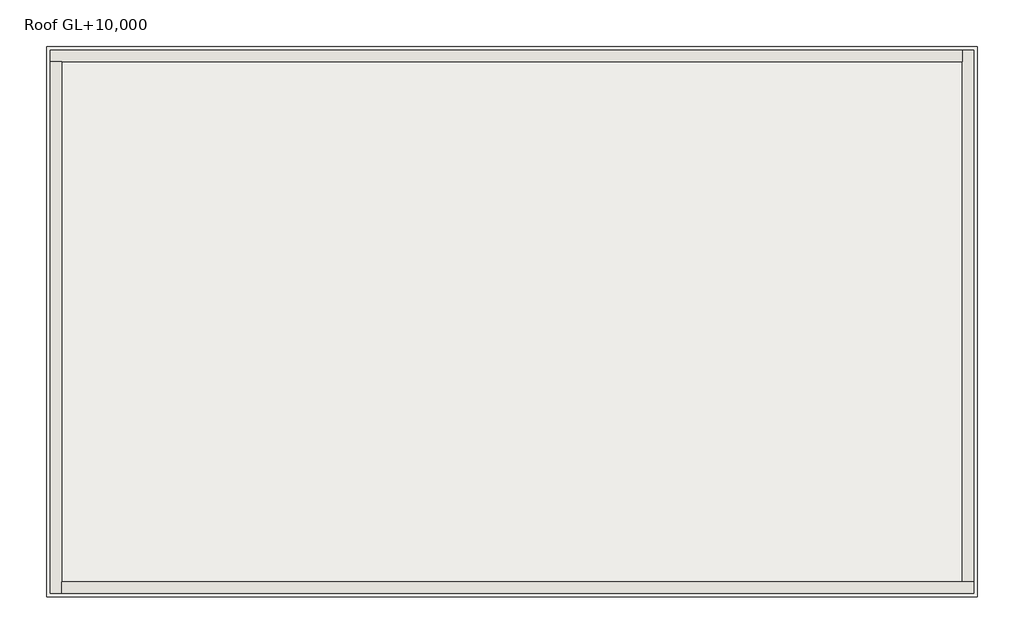
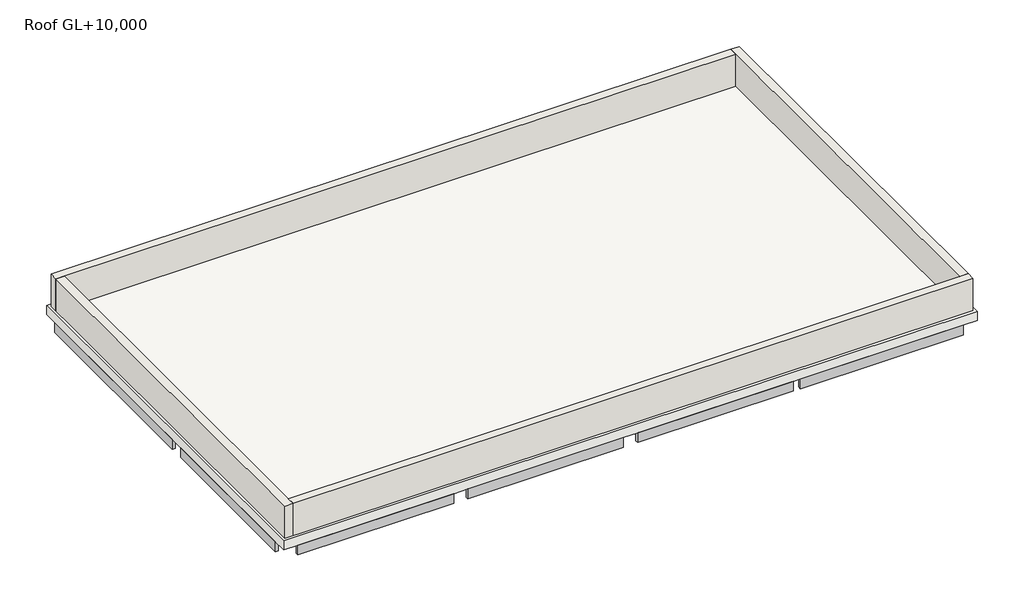
# One storey: 22 beams, 4 walls, 1 roof.
"""IFC4 building model written with IfcOpenShell, lengths in millimetres."""

import ifcopenshell
import ifcopenshell.guid

model = None  # the IFC model being written
_history = None  # IfcOwnerHistory: only IFC2X3 demands one
_inside = {}  # id of a spatial element -> (the spatial element, [elements in it])
_under = {}  # id of a project, library or spatial element -> (it, [spatial elements below it])
_declared = {}  # id of a project -> (the project, [libraries it declares])
_typed = {}  # id of a type object -> (the type object, [elements of that type])
_made_of = {}  # id of a material, layer set ... -> (it, [elements and type objects made of it])


def new_model(schema):
    """Start an empty IFC model of exactly this schema.

    Asked for "IFC4X3", IfcOpenShell would pick the latest addendum, in which some entities
    have other attributes; the version numbers below select the first issue.
    IFC2X3 requires an IfcOwnerHistory on every rooted entity: one is made here for all.
    """
    global model, _history
    if schema == "IFC4X3":
        model = ifcopenshell.file(schema_version=(4, 3, 0, 0))
    else:
        model = ifcopenshell.file(schema=schema)
    _inside.clear()
    _under.clear()
    _declared.clear()
    _typed.clear()
    _made_of.clear()
    _history = None
    if model.schema == "IFC2X3":
        org = make("IfcOrganization", Name="unknown")
        user = make(
            "IfcPersonAndOrganization",
            ThePerson=make("IfcPerson", FamilyName="unknown"),
            TheOrganization=org,
        )
        app = make(
            "IfcApplication",
            ApplicationDeveloper=org,
            Version="unknown",
            ApplicationFullName="unknown",
            ApplicationIdentifier="unknown",
        )
        _history = make(
            "IfcOwnerHistory",
            OwningUser=user,
            OwningApplication=app,
            ChangeAction="ADDED",
            CreationDate=0,
        )
    return model


def make(cls, **values):
    """One entity of the class cls with the attributes given. An attribute that is None is left unset."""
    return model.create_entity(
        cls, **{name: value for name, value in values.items() if value is not None}
    )


def rooted(cls, **values):
    """An entity with a GlobalId (a new one), such as an element, a storey or a relation."""
    return make(cls, GlobalId=ifcopenshell.guid.new(), OwnerHistory=_history, **values)


def si_unit(unit_type, name, prefix=None):
    """IfcSIUnit, for example si_unit("LENGTHUNIT", "METRE", prefix="MILLI")."""
    return make("IfcSIUnit", UnitType=unit_type, Prefix=prefix, Name=name)


def assignment(units):
    """IfcUnitAssignment: the units of a project."""
    return None if units is None else make("IfcUnitAssignment", Units=units)


def point(xyz):
    """IfcCartesianPoint."""
    return None if xyz is None else make("IfcCartesianPoint", Coordinates=xyz)


def direction(xyz):
    """IfcDirection."""
    return None if xyz is None else make("IfcDirection", DirectionRatios=xyz)


def frame(location, z_axis=None, x_axis=None):
    """IfcAxis2Placement3D, a coordinate frame: its origin and axes. An axis left out is left unset."""
    return make(
        "IfcAxis2Placement3D",
        Location=point(location),
        Axis=direction(z_axis),
        RefDirection=direction(x_axis),
    )


def origin():
    """The frame at (0, 0, 0) with its axes left unset."""
    return frame((0.0, 0.0, 0.0))


def place(relative_to, where):
    """IfcLocalPlacement: puts the frame where relative to a parent placement (None: the world)."""
    return make(
        "IfcLocalPlacement", PlacementRelTo=relative_to, RelativePlacement=where
    )


def context(
    kind, dimensions, precision=None, world=None, true_north=None, identifier=None
):
    """IfcGeometricRepresentationContext, for example the 3D "Model" context."""
    return make(
        "IfcGeometricRepresentationContext",
        ContextIdentifier=identifier,
        ContextType=kind,
        CoordinateSpaceDimension=dimensions,
        Precision=precision,
        WorldCoordinateSystem=world,
        TrueNorth=true_north,
    )


def project(units=None, contexts=None):
    """IfcProject with its units and contexts."""
    return rooted(
        "IfcProject",
        Name="project",
        RepresentationContexts=contexts,
        UnitsInContext=assignment(units),
    )


def spatial(cls, under=None, at=None, **own):
    """A site, building, storey or space (cls), placed at a placement, below another one or the project."""
    s = rooted(cls, ObjectPlacement=at, **own)
    if under is not None:
        _under.setdefault(under.id(), (under, []))[1].append(s)
    return s


def polyline(points):
    """IfcPolyline through the points."""
    return make("IfcPolyline", Points=[point(p) for p in points])


def outline(outer, holes=None, kind="AREA"):
    """IfcArbitraryClosedProfileDef: a profile drawn as a closed curve; with holes, ...WithVoids."""
    if holes is None:
        return make("IfcArbitraryClosedProfileDef", ProfileType=kind, OuterCurve=outer)
    return make(
        "IfcArbitraryProfileDefWithVoids",
        ProfileType=kind,
        OuterCurve=outer,
        InnerCurves=holes,
    )


def extrude(swept, where, along, depth):
    """IfcExtrudedAreaSolid: the profile swept, set in the frame where, extruded along a direction by depth."""
    return make(
        "IfcExtrudedAreaSolid",
        SweptArea=swept,
        Position=where,
        ExtrudedDirection=direction(along),
        Depth=depth,
    )


def faces_of(points, faces, orient=None, outer=None):
    """IfcFace entities. A face is a list of loops; a loop is a list of indices into points, from 0.

    orient and outer hold one flag for each loop. By default every Orientation is true, the
    first loop of a face is its IfcFaceOuterBound and the others are IfcFaceBound.
    """
    made = []
    for i, loops in enumerate(faces):
        bounds = []
        for j, loop in enumerate(loops):
            is_outer = j == 0 if outer is None else outer[i][j]
            bounds.append(
                make(
                    "IfcFaceOuterBound" if is_outer else "IfcFaceBound",
                    Bound=make("IfcPolyLoop", Polygon=[points[k] for k in loop]),
                    Orientation=True if orient is None else orient[i][j],
                )
            )
        made.append(make("IfcFace", Bounds=bounds))
    return made


def faceted_brep(points, faces, orient=None, outer=None, voids=None):
    """IfcFacetedBrep: a solid bounded by flat faces; with voids (closed shells), ...WithVoids."""
    shared = [point(p) for p in points]
    hull = make("IfcClosedShell", CfsFaces=faces_of(shared, faces, orient, outer))
    if voids is None:
        return make("IfcFacetedBrep", Outer=hull)
    return make(
        "IfcFacetedBrepWithVoids",
        Outer=hull,
        Voids=[
            make(cls, CfsFaces=faces_of(shared, fs, o, b)) for cls, fs, o, b in voids
        ],
    )


def shape(context_of_items, identifier, shape_type, items):
    """IfcShapeRepresentation: the items that make up one representation, for example the "Body"."""
    return make(
        "IfcShapeRepresentation",
        ContextOfItems=context_of_items,
        RepresentationIdentifier=identifier,
        RepresentationType=shape_type,
        Items=items,
    )


def made_of(thing, what):
    """Note that an element or type object is made of a material, layer set ...; save() writes the relation."""
    if what is not None:
        _made_of.setdefault(what.id(), (what, []))[1].append(thing)
    return thing


def element(
    cls,
    number,
    at=None,
    inside=None,
    cuts=None,
    type_object=None,
    material=None,
    context=None,
    identifier="Body",
    shape_type=None,
    held_by="IfcProductDefinitionShape",
    body=None,
    shapes=None,
    **own,
):
    """One element of the class cls, such as IfcWall. Its Tag is "e" and its number.

    at: its placement. inside: the storey or other place that contains it. cuts: it is an
    opening in that element (IfcRelVoidsElement). A single representation is given by context,
    identifier, shape_type and body (its items); several are given by shapes. held_by: the class
    of the entity that holds the representations. save() writes the other relations.
    """
    e = rooted(cls, Tag="e%d" % number, ObjectPlacement=at, **own)
    if body is not None:
        shapes = [shape(context, identifier, shape_type, body)]
    if shapes is not None:
        e.Representation = make(held_by, Representations=shapes)
    if inside is not None:
        _inside.setdefault(inside.id(), (inside, []))[1].append(e)
    if cuts is not None:
        rooted(
            "IfcRelVoidsElement", RelatingBuildingElement=cuts, RelatedOpeningElement=e
        )
    if type_object is not None:
        _typed.setdefault(type_object.id(), (type_object, []))[1].append(e)
    return made_of(e, material)


def aggregate(whole, parts):
    """IfcRelAggregates: a whole, such as a stair, and the parts it consists of."""
    return rooted("IfcRelAggregates", RelatingObject=whole, RelatedObjects=parts)


def save(model, path):
    """Write the relations noted so far, then the file.

    IfcRelAggregates (storeys below a building ...), IfcRelContainedInSpatialStructure (elements
    in a storey), IfcRelDefinesByType, IfcRelAssociatesMaterial and IfcRelDeclares: one each for
    every whole, place, type object, material and project.
    """
    for whole, parts in _under.values():
        aggregate(whole, parts)
    for where, things in _inside.values():
        rooted(
            "IfcRelContainedInSpatialStructure",
            RelatedElements=things,
            RelatingStructure=where,
        )
    for kind, things in _typed.values():
        rooted("IfcRelDefinesByType", RelatedObjects=things, RelatingType=kind)
    for what, things in _made_of.values():
        rooted("IfcRelAssociatesMaterial", RelatedObjects=things, RelatingMaterial=what)
    for by, libraries in _declared.values():
        rooted("IfcRelDeclares", RelatingContext=by, RelatedDefinitions=libraries)
    model.write(path)


model = new_model("IFC4")

# Units and contexts
model_context = context("Model", 3, world=origin())
ifc_project = project(units=[si_unit("LENGTHUNIT", "METRE", prefix="MILLI")], contexts=[model_context])

# Site, building, storey
site = spatial("IfcSite", under=ifc_project)
building = spatial("IfcBuilding", under=site)
storey = spatial("IfcBuildingStorey", under=building, Name="Roof GL+10,000", Elevation=10000.0)

# Beams
placement = place(None, origin())
element("IfcBeam", 1, ObjectType="RC Beam_Rectangular : 350 x 700mm", at=placement, inside=storey, context=model_context, shape_type="SweptSolid", body=[
    extrude(outline(polyline([(-18945.7273237, -4314.0236875), (-18945.7273237, 1485.9763125), (-18845.7273237, 1485.9763125), (-18845.7273237, -4314.0236875), (-18945.7273237, -4314.0236875)])), frame((0.0, 0.0, 9300.0), z_axis=(0.0, 0.0, 1.0), x_axis=(1.0, 0.0, 0.0)), (0.0, 0.0, 1.0), 367.0),
])
element("IfcBeam", 2, ObjectType="RC Beam_Rectangular : 350 x 700mm", at=placement, inside=storey, context=model_context, shape_type="SweptSolid", body=[
    extrude(outline(polyline([(-18945.7273237, 1998.6763125), (-18945.7273237, 9185.9763125), (-18845.7273237, 9185.9763125), (-18845.7273237, 1998.6763125), (-18945.7273237, 1998.6763125)])), frame((0.0, 0.0, 9300.0), z_axis=(0.0, 0.0, 1.0), x_axis=(1.0, 0.0, 0.0)), (0.0, 0.0, 1.0), 367.0),
])
element("IfcBeam", 3, ObjectType="RC Beam_Rectangular : 350 x 700mm", at=placement, inside=storey, context=model_context, shape_type="SweptSolid", body=[
    extrude(outline(polyline([(-12520.7273237, 1485.9763125), (-12520.7273237, -4314.0236875), (-12545.7273237, -4314.0236875), (-12545.7273237, 1485.9763125), (-12520.7273237, 1485.9763125)])), frame((0.0, 0.0, 9300.0), z_axis=(0.0, 0.0, 1.0), x_axis=(1.0, 0.0, 0.0)), (0.0, 0.0, 1.0), 367.0),
    extrude(outline(polyline([(-12870.7273237, -4314.0236875), (-12870.7273237, 1485.9763125), (-12845.7273237, 1485.9763125), (-12845.7273237, -4314.0236875), (-12870.7273237, -4314.0236875)])), frame((0.0, 0.0, 9300.0), z_axis=(0.0, 0.0, 1.0), x_axis=(1.0, 0.0, 0.0)), (0.0, 0.0, 1.0), 367.0),
])
element("IfcBeam", 4, ObjectType="RC Beam_Rectangular : 350 x 700mm", at=placement, inside=storey, context=model_context, shape_type="SweptSolid", body=[
    extrude(outline(polyline([(-12870.7273237, 9185.9763125), (-12520.7273237, 9185.9763125), (-12520.7273237, 1985.9763125), (-12870.7273237, 1985.9763125), (-12870.7273237, 9185.9763125)])), frame((0.0, 0.0, 9300.0), z_axis=(0.0, 0.0, 1.0), x_axis=(1.0, 0.0, 0.0)), (0.0, 0.0, 1.0), 367.0),
])
element("IfcBeam", 5, ObjectType="RC Beam_Rectangular : 350 x 700mm", at=placement, inside=storey, context=model_context, shape_type="SweptSolid", body=[
    extrude(outline(polyline([(-6520.7273237, 1485.9763125), (-6520.7273237, -4314.0236875), (-6545.7273237, -4314.0236875), (-6545.7273237, 1485.9763125), (-6520.7273237, 1485.9763125)])), frame((0.0, 0.0, 9300.0), z_axis=(0.0, 0.0, 1.0), x_axis=(1.0, 0.0, 0.0)), (0.0, 0.0, 1.0), 367.0),
    extrude(outline(polyline([(-6870.7273237, -4314.0236875), (-6870.7273237, 1485.9763125), (-6845.7273237, 1485.9763125), (-6845.7273237, -4314.0236875), (-6870.7273237, -4314.0236875)])), frame((0.0, 0.0, 9300.0), z_axis=(0.0, 0.0, 1.0), x_axis=(1.0, 0.0, 0.0)), (0.0, 0.0, 1.0), 367.0),
])
element("IfcBeam", 6, ObjectType="RC Beam_Rectangular : 350 x 700mm", at=placement, inside=storey, context=model_context, shape_type="SweptSolid", body=[
    extrude(outline(polyline([(-6520.7273237, 3985.9763125), (-6520.7273237, 1985.9763125), (-6545.7273237, 1985.9763125), (-6545.7273237, 3985.9763125), (-6520.7273237, 3985.9763125)])), frame((0.0, 0.0, 9300.0), z_axis=(0.0, 0.0, 1.0), x_axis=(1.0, 0.0, 0.0)), (0.0, 0.0, 1.0), 367.0),
    extrude(outline(polyline([(-6870.7273237, 1985.9763125), (-6870.7273237, 3985.9763125), (-6845.7273237, 3985.9763125), (-6845.7273237, 1985.9763125), (-6870.7273237, 1985.9763125)])), frame((0.0, 0.0, 9300.0), z_axis=(0.0, 0.0, 1.0), x_axis=(1.0, 0.0, 0.0)), (0.0, 0.0, 1.0), 367.0),
    extrude(outline(polyline([(-6870.7273237, 9185.9763125), (-6520.7273237, 9185.9763125), (-6520.7273237, 4285.9763125), (-6870.7273237, 4285.9763125), (-6870.7273237, 9185.9763125)])), frame((0.0, 0.0, 9300.0), z_axis=(0.0, 0.0, 1.0), x_axis=(1.0, 0.0, 0.0)), (0.0, 0.0, 1.0), 367.0),
])
element("IfcBeam", 7, ObjectType="RC Beam_Rectangular : 350 x 700mm", at=placement, inside=storey, context=model_context, shape_type="SweptSolid", body=[
    extrude(outline(polyline([(-520.7273237, 1485.9763125), (-520.7273237, -4314.0236875), (-545.7273237, -4314.0236875), (-545.7273237, 1485.9763125), (-520.7273237, 1485.9763125)])), frame((0.0, 0.0, 9300.0), z_axis=(0.0, 0.0, 1.0), x_axis=(1.0, 0.0, 0.0)), (0.0, 0.0, 1.0), 367.0),
    extrude(outline(polyline([(-870.7273237, -4314.0236875), (-870.7273237, 1485.9763125), (-845.7273237, 1485.9763125), (-845.7273237, -4314.0236875), (-870.7273237, -4314.0236875)])), frame((0.0, 0.0, 9300.0), z_axis=(0.0, 0.0, 1.0), x_axis=(1.0, 0.0, 0.0)), (0.0, 0.0, 1.0), 367.0),
])
element("IfcBeam", 8, ObjectType="RC Beam_Rectangular : 350 x 700mm", at=placement, inside=storey, context=model_context, shape_type="SweptSolid", body=[
    extrude(outline(polyline([(-520.7273237, 1985.9763125), (-870.7273237, 1985.9763125), (-870.7273237, 3985.9763125), (-520.7273237, 3985.9763125), (-520.7273237, 1985.9763125)])), frame((0.0, 0.0, 9300.0), z_axis=(0.0, 0.0, 1.0), x_axis=(1.0, 0.0, 0.0)), (0.0, 0.0, 1.0), 367.0),
    extrude(outline(polyline([(-870.7273237, 9185.9763125), (-520.7273237, 9185.9763125), (-520.7273237, 4285.9763125), (-870.7273237, 4285.9763125), (-870.7273237, 9185.9763125)])), frame((0.0, 0.0, 9300.0), z_axis=(0.0, 0.0, 1.0), x_axis=(1.0, 0.0, 0.0)), (0.0, 0.0, 1.0), 367.0),
])
element("IfcBeam", 9, ObjectType="RC Beam_Rectangular : 350 x 700mm", at=placement, inside=storey, context=model_context, shape_type="SweptSolid", body=[
    extrude(outline(polyline([(5554.2726763, 1485.9763125), (5554.2726763, -4314.0236875), (5454.2726763, -4314.0236875), (5454.2726763, 1485.9763125), (5554.2726763, 1485.9763125)])), frame((0.0, 0.0, 9300.0), z_axis=(0.0, 0.0, 1.0), x_axis=(1.0, 0.0, 0.0)), (0.0, 0.0, 1.0), 367.0),
])
element("IfcBeam", 10, ObjectType="RC Beam_Rectangular : 350 x 700mm", at=placement, inside=storey, context=model_context, shape_type="SweptSolid", body=[
    extrude(outline(polyline([(5554.2726763, 9185.9763125), (5554.2726763, 1998.6763125), (5454.2726763, 1998.6763125), (5454.2726763, 9185.9763125), (5554.2726763, 9185.9763125)])), frame((0.0, 0.0, 9300.0), z_axis=(0.0, 0.0, 1.0), x_axis=(1.0, 0.0, 0.0)), (0.0, 0.0, 1.0), 367.0),
])
element("IfcBeam", 11, ObjectType="RC Beam_Rectangular : 350 x 700mm", at=placement, inside=storey, context=model_context, shape_type="SweptSolid", body=[
    extrude(outline(polyline([(-18445.7273237, 9685.9763125), (-12945.7273237, 9685.9763125), (-12945.7273237, 9585.9763125), (-18445.7273237, 9585.9763125), (-18445.7273237, 9685.9763125)])), frame((0.0, 0.0, 9300.0), z_axis=(0.0, 0.0, 1.0), x_axis=(1.0, 0.0, 0.0)), (0.0, 0.0, 1.0), 367.0),
])
element("IfcBeam", 12, ObjectType="RC Beam_Rectangular : 350 x 700mm", at=placement, inside=storey, context=model_context, shape_type="SweptSolid", body=[
    extrude(outline(polyline([(-12445.7273237, 9685.9763125), (-6945.7273237, 9685.9763125), (-6945.7273237, 9585.9763125), (-12445.7273237, 9585.9763125), (-12445.7273237, 9685.9763125)])), frame((0.0, 0.0, 9300.0), z_axis=(0.0, 0.0, 1.0), x_axis=(1.0, 0.0, 0.0)), (0.0, 0.0, 1.0), 367.0),
])
element("IfcBeam", 13, ObjectType="RC Beam_Rectangular : 350 x 700mm", at=placement, inside=storey, context=model_context, shape_type="SweptSolid", body=[
    extrude(outline(polyline([(-6445.7273237, 9685.9763125), (-945.7273237, 9685.9763125), (-945.7273237, 9585.9763125), (-6445.7273237, 9585.9763125), (-6445.7273237, 9685.9763125)])), frame((0.0, 0.0, 9300.0), z_axis=(0.0, 0.0, 1.0), x_axis=(1.0, 0.0, 0.0)), (0.0, 0.0, 1.0), 367.0),
])
element("IfcBeam", 14, ObjectType="RC Beam_Rectangular : 350 x 700mm", at=placement, inside=storey, context=model_context, shape_type="SweptSolid", body=[
    extrude(outline(polyline([(-445.7273237, 9685.9763125), (5054.2726763, 9685.9763125), (5054.2726763, 9585.9763125), (-445.7273237, 9585.9763125), (-445.7273237, 9685.9763125)])), frame((0.0, 0.0, 9300.0), z_axis=(0.0, 0.0, 1.0), x_axis=(1.0, 0.0, 0.0)), (0.0, 0.0, 1.0), 367.0),
])
element("IfcBeam", 15, ObjectType="RC Beam_Rectangular : 350 x 700mm", at=placement, inside=storey, context=model_context, shape_type="SweptSolid", body=[
    extrude(outline(polyline([(-12945.7273237, 1560.9763125), (-18445.7273237, 1560.9763125), (-18445.7273237, 1585.9763125), (-12945.7273237, 1585.9763125), (-12945.7273237, 1560.9763125)])), frame((0.0, 0.0, 9300.0), z_axis=(0.0, 0.0, 1.0), x_axis=(1.0, 0.0, 0.0)), (0.0, 0.0, 1.0), 367.0),
    extrude(outline(polyline([(-18445.7273237, 1910.9763125), (-12945.7273237, 1910.9763125), (-12945.7273237, 1885.9763125), (-18445.7273237, 1885.9763125), (-18445.7273237, 1910.9763125)])), frame((0.0, 0.0, 9300.0), z_axis=(0.0, 0.0, 1.0), x_axis=(1.0, 0.0, 0.0)), (0.0, 0.0, 1.0), 367.0),
])
element("IfcBeam", 16, ObjectType="RC Beam_Rectangular : 350 x 700mm", at=placement, inside=storey, context=model_context, shape_type="SweptSolid", body=[
    extrude(outline(polyline([(-6945.7273237, 1560.9763125), (-12445.7273237, 1560.9763125), (-12445.7273237, 1585.9763125), (-6945.7273237, 1585.9763125), (-6945.7273237, 1560.9763125)])), frame((0.0, 0.0, 9300.0), z_axis=(0.0, 0.0, 1.0), x_axis=(1.0, 0.0, 0.0)), (0.0, 0.0, 1.0), 367.0),
    extrude(outline(polyline([(-12445.7273237, 1910.9763125), (-6945.7273237, 1910.9763125), (-6945.7273237, 1885.9763125), (-12445.7273237, 1885.9763125), (-12445.7273237, 1910.9763125)])), frame((0.0, 0.0, 9300.0), z_axis=(0.0, 0.0, 1.0), x_axis=(1.0, 0.0, 0.0)), (0.0, 0.0, 1.0), 367.0),
])
element("IfcBeam", 17, ObjectType="RC Beam_Rectangular : 350 x 700mm", at=placement, inside=storey, context=model_context, shape_type="SweptSolid", body=[
    extrude(outline(polyline([(-945.7273237, 1585.9763125), (-945.7273237, 1560.9763125), (-6445.7273237, 1560.9763125), (-6445.7273237, 1585.9763125), (-945.7273237, 1585.9763125)])), frame((0.0, 0.0, 9300.0), z_axis=(0.0, 0.0, 1.0), x_axis=(1.0, 0.0, 0.0)), (0.0, 0.0, 1.0), 367.0),
    extrude(outline(polyline([(-945.7273237, 1910.9763125), (-945.7273237, 1885.9763125), (-6445.7273237, 1885.9763125), (-6445.7273237, 1910.9763125), (-945.7273237, 1910.9763125)])), frame((0.0, 0.0, 9300.0), z_axis=(0.0, 0.0, 1.0), x_axis=(1.0, 0.0, 0.0)), (0.0, 0.0, 1.0), 367.0),
])
element("IfcBeam", 18, ObjectType="RC Beam_Rectangular : 350 x 700mm", at=placement, inside=storey, context=model_context, shape_type="SweptSolid", body=[
    extrude(outline(polyline([(-445.7273237, 1560.9763125), (-445.7273237, 1585.9763125), (2154.2726763, 1585.9763125), (2154.2726763, 1560.9763125), (-445.7273237, 1560.9763125)])), frame((0.0, 0.0, 9300.0), z_axis=(0.0, 0.0, 1.0), x_axis=(1.0, 0.0, 0.0)), (0.0, 0.0, 1.0), 367.0),
    extrude(outline(polyline([(-445.7273237, 1910.9763125), (5054.2726763, 1910.9763125), (5054.2726763, 1885.9763125), (-445.7273237, 1885.9763125), (-445.7273237, 1910.9763125)])), frame((0.0, 0.0, 9300.0), z_axis=(0.0, 0.0, 1.0), x_axis=(1.0, 0.0, 0.0)), (0.0, 0.0, 1.0), 367.0),
    extrude(outline(polyline([(5054.2726763, 1585.9763125), (5054.2726763, 1560.9763125), (2454.2726763, 1560.9763125), (2454.2726763, 1585.9763125), (5054.2726763, 1585.9763125)])), frame((0.0, 0.0, 9300.0), z_axis=(0.0, 0.0, 1.0), x_axis=(1.0, 0.0, 0.0)), (0.0, 0.0, 1.0), 367.0),
])
element("IfcBeam", 19, ObjectType="RC Beam_Rectangular : 350 x 700mm", at=placement, inside=storey, context=model_context, shape_type="SweptSolid", body=[
    extrude(outline(polyline([(-12945.7273237, -4814.0236875), (-18445.7273237, -4814.0236875), (-18445.7273237, -4714.0236875), (-12945.7273237, -4714.0236875), (-12945.7273237, -4814.0236875)])), frame((0.0, 0.0, 9300.0), z_axis=(0.0, 0.0, 1.0), x_axis=(1.0, 0.0, 0.0)), (0.0, 0.0, 1.0), 367.0),
])
element("IfcBeam", 20, ObjectType="RC Beam_Rectangular : 350 x 700mm", at=placement, inside=storey, context=model_context, shape_type="SweptSolid", body=[
    extrude(outline(polyline([(-6945.7273237, -4714.0236875), (-6945.7273237, -4814.0236875), (-12445.7273237, -4814.0236875), (-12445.7273237, -4714.0236875), (-6945.7273237, -4714.0236875)])), frame((0.0, 0.0, 9300.0), z_axis=(0.0, 0.0, 1.0), x_axis=(1.0, 0.0, 0.0)), (0.0, 0.0, 1.0), 367.0),
])
element("IfcBeam", 21, ObjectType="RC Beam_Rectangular : 350 x 700mm", at=placement, inside=storey, context=model_context, shape_type="SweptSolid", body=[
    extrude(outline(polyline([(-945.7273237, -4714.0236875), (-945.7273237, -4814.0236875), (-6445.7273237, -4814.0236875), (-6445.7273237, -4714.0236875), (-945.7273237, -4714.0236875)])), frame((0.0, 0.0, 9300.0), z_axis=(0.0, 0.0, 1.0), x_axis=(1.0, 0.0, 0.0)), (0.0, 0.0, 1.0), 367.0),
])
element("IfcBeam", 22, ObjectType="RC Beam_Rectangular : 350 x 700mm", at=placement, inside=storey, context=model_context, shape_type="SweptSolid", body=[
    extrude(outline(polyline([(5054.2726763, -4814.0236875), (-695.7273237, -4814.0236875), (-695.7273237, -4714.0236875), (5054.2726763, -4714.0236875), (5054.2726763, -4814.0236875)])), frame((0.0, 0.0, 9300.0), z_axis=(0.0, 0.0, 1.0), x_axis=(1.0, 0.0, 0.0)), (0.0, 0.0, 1.0), 367.0),
])

# Roof
element("IfcRoof", 23, ObjectType="H_RF_AMRF_Membrane_Insulation_Protection", at=placement, inside=storey, context=model_context, shape_type="Brep", body=[
    faceted_brep([(5554.2726763, 9685.9763125, 9667.0), (5554.2726763, 9185.9763125, 9667.0), (5554.2726763, 1998.6763125, 9667.0), (5554.2726763, 1985.9763125, 9667.0), (5554.2726763, 1485.9763125, 9667.0), (5554.2726763, -4314.0236875, 9667.0), (5554.2726763, -4814.0236875, 9667.0), (5054.2726763, -4814.0236875, 9667.0), (-445.7273237, -4814.0236875, 9667.0), (-695.7273237, -4814.0236875, 9667.0), (-945.7273237, -4814.0236875, 9667.0), (-6445.7273237, -4814.0236875, 9667.0), (-6945.7273237, -4814.0236875, 9667.0), (-12445.7273237, -4814.0236875, 9667.0), (-12945.7273237, -4814.0236875, 9667.0), (-18445.7273237, -4814.0236875, 9667.0), (-18945.7273237, -4814.0236875, 9667.0), (-18945.7273237, -4314.0236875, 9667.0), (-18945.7273237, 1485.9763125, 9667.0), (-18945.7273237, 1985.9763125, 9667.0), (-18945.7273237, 1998.6763125, 9667.0), (-18945.7273237, 9185.9763125, 9667.0), (-18945.7273237, 9685.9763125, 9667.0), (-18445.7273237, 9685.9763125, 9667.0), (-12945.7273237, 9685.9763125, 9667.0), (-12445.7273237, 9685.9763125, 9667.0), (-6945.7273237, 9685.9763125, 9667.0), (-6445.7273237, 9685.9763125, 9667.0), (-945.7273237, 9685.9763125, 9667.0), (-445.7273237, 9685.9763125, 9667.0), (5054.2726763, 9685.9763125, 9667.0), (5554.2726763, -4814.0236875, 10000.0), (5554.2726763, 9685.9763125, 10000.0), (-18945.7273237, 9685.9763125, 10000.0), (-18945.7273237, -4814.0236875, 10000.0)], [[[0, 1, 2, 3, 4, 5, 6, 7, 8, 9, 10, 11, 12, 13, 14, 15, 16, 17, 18, 19, 20, 21, 22, 23, 24, 25, 26, 27, 28, 29, 30]], [[31, 32, 33, 34]], [[32, 31, 6, 5, 4, 3, 2, 1, 0]], [[33, 32, 0, 30, 29, 28, 27, 26, 25, 24, 23, 22]], [[34, 33, 22, 21, 20, 19, 18, 17, 16]], [[31, 34, 16, 15, 14, 13, 12, 11, 10, 9, 8, 7, 6]]]),
])

# Walls
element("IfcWall", 24, ObjectType="일반 - 300mm", at=placement, inside=storey, context=model_context, shape_type="Brep", body=[
    faceted_brep([(-18845.7273237, 9285.9763125, 10000.0), (-18545.7273237, 9285.9763125, 10000.0), (5154.2726763, 9285.9763125, 10000.0), (5154.2726763, 9285.9763125, 11200.0), (-18545.7273237, 9285.9763125, 11200.0), (-18845.7273237, 9285.9763125, 11200.0), (-18845.7273237, 9585.9763125, 10000.0), (-18845.7273237, 9585.9763125, 11200.0), (5154.2726763, 9585.9763125, 11200.0), (5154.2726763, 9585.9763125, 10000.0)], [[[0, 1, 2, 3, 4, 5]], [[6, 7, 8, 9]], [[2, 1, 0, 6, 9]], [[5, 4, 3, 8, 7]], [[0, 5, 7, 6]], [[3, 2, 9, 8]]]),
])
element("IfcWall", 25, ObjectType="일반 - 300mm", at=placement, inside=storey, context=model_context, shape_type="Brep", body=[
    faceted_brep([(-18545.7273237, -4714.0236875, 10000.0), (-18545.7273237, -4414.0236875, 10000.0), (-18545.7273237, 9285.9763125, 10000.0), (-18545.7273237, 9285.9763125, 11200.0), (-18545.7273237, -4414.0236875, 11200.0), (-18545.7273237, -4714.0236875, 11200.0), (-18845.7273237, -4714.0236875, 10000.0), (-18845.7273237, -4714.0236875, 11200.0), (-18845.7273237, 9285.9763125, 11200.0), (-18845.7273237, 9285.9763125, 10000.0)], [[[0, 1, 2, 3, 4, 5]], [[6, 7, 8, 9]], [[2, 1, 0, 6, 9]], [[5, 4, 3, 8, 7]], [[0, 5, 7, 6]], [[3, 2, 9, 8]]]),
])
element("IfcWall", 26, ObjectType="일반 - 300mm", at=placement, inside=storey, context=model_context, shape_type="Brep", body=[
    faceted_brep([(5454.2726763, -4414.0236875, 10000.0), (5154.2726763, -4414.0236875, 10000.0), (-18545.7273237, -4414.0236875, 10000.0), (-18545.7273237, -4414.0236875, 11200.0), (5154.2726763, -4414.0236875, 11200.0), (5454.2726763, -4414.0236875, 11200.0), (5454.2726763, -4714.0236875, 10000.0), (5454.2726763, -4714.0236875, 11200.0), (-18545.7273237, -4714.0236875, 11200.0), (-18545.7273237, -4714.0236875, 10000.0)], [[[0, 1, 2, 3, 4, 5]], [[6, 7, 8, 9]], [[2, 1, 0, 6, 9]], [[5, 4, 3, 8, 7]], [[0, 5, 7, 6]], [[3, 2, 9, 8]]]),
])
element("IfcWall", 27, ObjectType="일반 - 300mm", at=placement, inside=storey, context=model_context, shape_type="Brep", body=[
    faceted_brep([(5154.2726763, 9585.9763125, 10000.0), (5154.2726763, 9285.9763125, 10000.0), (5154.2726763, -4414.0236875, 10000.0), (5154.2726763, -4414.0236875, 11200.0), (5154.2726763, 9285.9763125, 11200.0), (5154.2726763, 9585.9763125, 11200.0), (5454.2726763, 9585.9763125, 10000.0), (5454.2726763, 9585.9763125, 11200.0), (5454.2726763, -4414.0236875, 11200.0), (5454.2726763, -4414.0236875, 10000.0)], [[[0, 1, 2, 3, 4, 5]], [[6, 7, 8, 9]], [[2, 1, 0, 6, 9]], [[5, 4, 3, 8, 7]], [[0, 5, 7, 6]], [[3, 2, 9, 8]]]),
])

save(model, "model.ifc")

# Revit data of these elements
# Type "RC Beam_Rectangular : 350 x 700mm"
#   Length [instance default] = 1524 mm
#   b = 350 mm
#   h = 700 mm
#   Structural Material [instance default] = 콘크리트, 현장타설 회색
#   Assembly Code = ""
# Type "H_RF_AMRF_Membrane_Insulation_Protection"
#   Layers, outside or top first: 38 mm "루핑, 타일" (function 4); 50 mm "고형 단열재" (function 3); 20 mm "아스팔트, 역청" (function 3); 0 mm "루핑 펠트" (function 100); 50 mm "콘크리트, 모래/시멘트 스크리드" (function 2); 175 mm "콘크리트, 현장치기" (function 1)
# Type "일반 - 300mm"
#   Layers, outside or top first: 300 mm no material (function 1)
# Elements 1, 2, 3, 4, 5, 6, 7, 8, 9, 10, 11, 12, 13, 14, 15, 16, 17, 18, 19, 20, 21, 22 (IfcBeam, "RC Beam_Rectangular : 350 x 700mm")
#   Structural Material = 콘크리트, 현장타설 회색
#   Phase Created = 신축
#   Materials on its faces: "콘크리트, 현장타설 회색"
# Element 23 (IfcRoof, "H_RF_AMRF_Membrane_Insulation_Protection")
#   Mark = "RF1"
#   Roof Base Material = "Concrete Slab"
#   Roof Finish_1 = "Light-Weight Concrete Screed (Slope 1%)"
#   Roof Finish_2 = "Waterproofing Membrane-EPDM(or Equivalent)"
#   Roof Finish_3 = "Rigid Extruded Polystyrene Foam Insulation(XPS)"
#   Roof Finish_4 = "PE Sheet (Vapor Barrier) 2Plies"
#   Roof Style Name = "Lightweight Concrete(Slope)+Waterproofing+Insulation+Protection Concrete"
#   Roof Finish_5 = "Protective Concrete w/ Steel Trowel Finish"
#   built-in parameter 1001705 = 32.8084 (stored number, unit not read)
#   built-in parameter 1001701 = -1.09252 (stored number, unit not read)
#   built-in parameter 1001710 = 33615
#   Roof Style = RF26
#   Phase Created = 신축
#   Materials on its faces: "콘크리트, 현장치기", "루핑, 타일"
# Elements 24, 25, 26, 27 (IfcWall, "일반 - 300mm")
#   Comments = ""
#   Wall Loca = "Parapet"
#   Top Offset = 0 mm
#   Base Offset = 0 mm
#   Unconnected Height = 1200 mm
#   wall height = 1200 mm
#   Phase Created = 신축
#   Base Constraint = Roof GL+10,000
#   Materials on its faces: "기본 벽"
# Materials
#   "콘크리트, 현장타설 회색": class "콘크리트", colour RGB 192 192 192, transparency 0, Description = "현장타설 콘크리트", Cost = 0
#   "루핑, 타일": class "금속", colour RGB 127 127 127, transparency 0, Description = "점토 루핑 타일", Cost = 0
#   "고형 단열재": class "일반", colour RGB 127 127 127, transparency 0, Description = "강체 폼 단열판", Cost = 0
#   "아스팔트, 역청": class "일반", colour RGB 155 155 155, transparency 0, Description = "역청 지붕 재료", Cost = 0
#   "루핑 펠트": class "일반", colour RGB 127 127 127, transparency 0, Description = "아스팔트 펠트", Cost = 0
#   "콘크리트, 모래/시멘트 스크리드": class "콘크리트", colour RGB 127 127 127, transparency 0, Description = "콘크리트 슬래브 덧침", Cost = 0
#   "콘크리트, 현장치기": class "콘크리트", colour RGB 192 192 192, transparency 0, Description = "물리적 재료", Cost = 0
#   "기본 벽": class "다양한", colour RGB 128 128 128, transparency 0, Cost = 0
